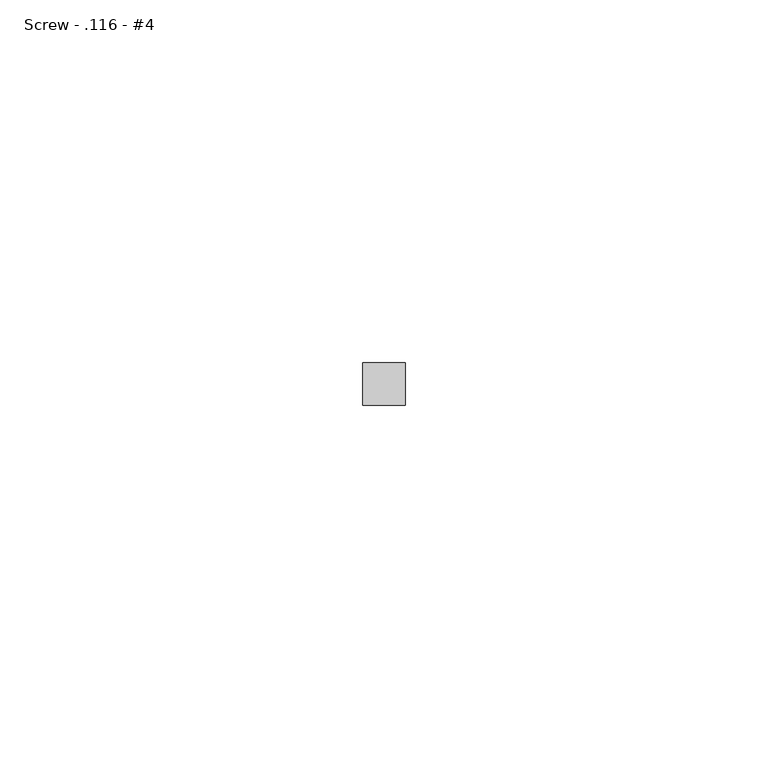
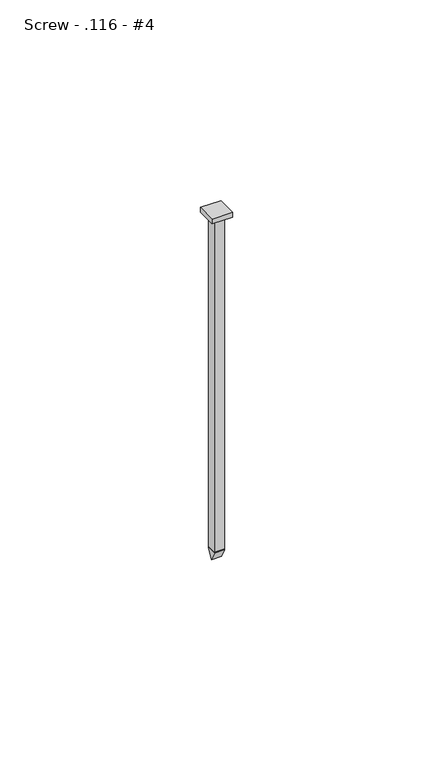
"""IFC4 building model written with IfcOpenShell, lengths in millimetres: fastener geometry, 060523 - W_P_C - Fastenings - Generic - SQUARE : Screw - .116 - #4."""

from ifc_helpers import new_model, si_unit, frame, origin, origin_with_axes, place, context, project, spatial, polyline, outline, extrude, source, transform, mapped, element, save


def screw_116_4_905c3a57(model_context):
    return source(origin(), model_context, "Body", "SweptSolid", [
        extrude(outline(polyline([(0.0, -104.5464), (-1.4732, -101.6), (1.4732, -101.6), (0.0, -104.5464)])), frame((-1.4732, 0.0, 0.0), z_axis=(1.0, 0.0, 0.0), x_axis=(0.0, 1.0, 0.0)), (0.0, 0.0, 1.0), 2.9464),
        extrude(outline(polyline([(-2.9464, -2.9464), (-2.9464, 2.9464), (2.9464, 2.9464), (2.9464, -2.9464), (-2.9464, -2.9464)])), origin_with_axes(), (0.0, 0.0, 1.0), 1.4732),
        extrude(outline(polyline([(-1.4732, 1.4732), (1.4732, 1.4732), (1.4732, -1.4732), (-1.4732, -1.4732), (-1.4732, 1.4732)])), frame((0.0, 0.0, -101.6), z_axis=(0.0, 0.0, 1.0), x_axis=(1.0, 0.0, 0.0)), (0.0, 0.0, 1.0), 101.6),
    ])


if __name__ == "__main__":
    model = new_model("IFC4")
    model_context = context("Model", 3, world=origin())
    ifc_project = project(units=[si_unit("LENGTHUNIT", "METRE", prefix="MILLI")], contexts=[model_context])
    site = spatial("IfcSite", under=ifc_project)
    building = spatial("IfcBuilding", under=site)
    placement = place(None, origin())
    screw_116_4_shape = screw_116_4_905c3a57(model_context)
    element("IfcFastener", 1, ObjectType="060523 - W_P_C - Fastenings - Generic - SQUARE : Screw - .116 - #4", at=placement, inside=building, context=model_context, shape_type="MappedRepresentation", body=[
        mapped(screw_116_4_shape, transform((0.0, 0.0, 0.0), x_axis=(1.0, 0.0, 0.0), y_axis=(0.0, 1.0, 0.0), z_axis=(0.0, 0.0, 1.0))),
    ])
    save(model, "model.ifc")

# Revit data of these elements
# Type "060523 - W_P_C - Fastenings - Generic - SQUARE : Screw - .116 - #4"
#   Washer_Thickness = 0' - 0.00333"
#   Washer Radius = 0' - 0.068"
#   Washer Offset - Head = 0' - 0"
#   Washer Offset = 0' - 0"
#   Thickness_of_Substrate [instance default] = 0' - 1"
#   Side = 0' - 0 37/64"
#   Radius = 0' - 0.058"
#   Length [instance default] = 0' - 4"
#   Head Size = 0' - 1"
#   Head Radius = 0' - 0 1/2"
#   Head Height = 0' - 0.01"
#   Double Diameter = 0' - 0.232"
#   Diameter = 0' - 0.116"
#   Default Elevation = 4' - 0"
#   Washer_Nut_Visibility = no
#   Washer_Head_Visibility = no
#   Round_Head_Visibility = yes
#   Point Visibility = yes
#   Nut_Visibility = no
#   Hex_Head_Visiblilty = no
#   Washer Material = none
#   Bolt Material (Size) = AT SILL - FASTENER AT 24" O.C.
# Materials
#   "AT SILL - FASTENER AT 24\" O.C.": class "Generic", colour RGB 120 120 120, transparency 0, Cost = 0
